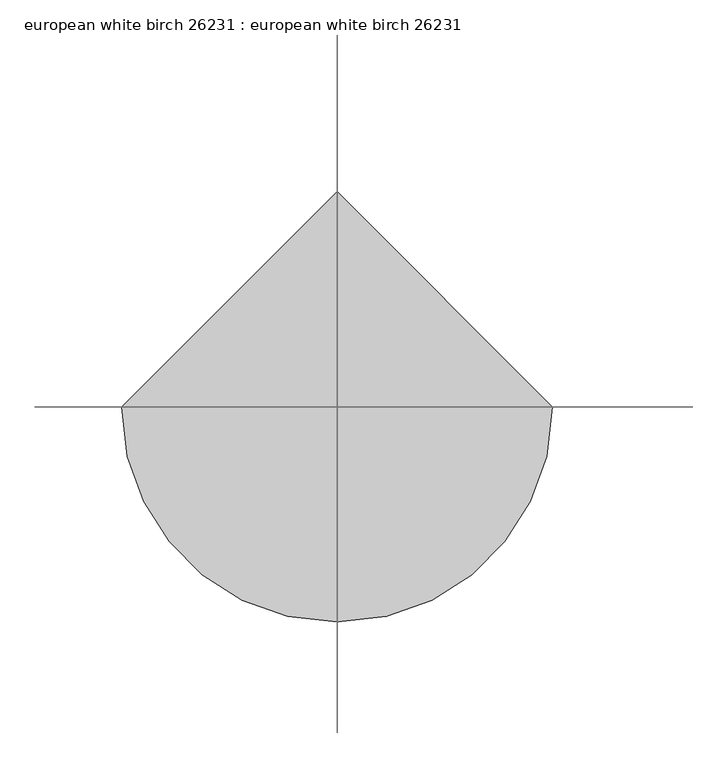
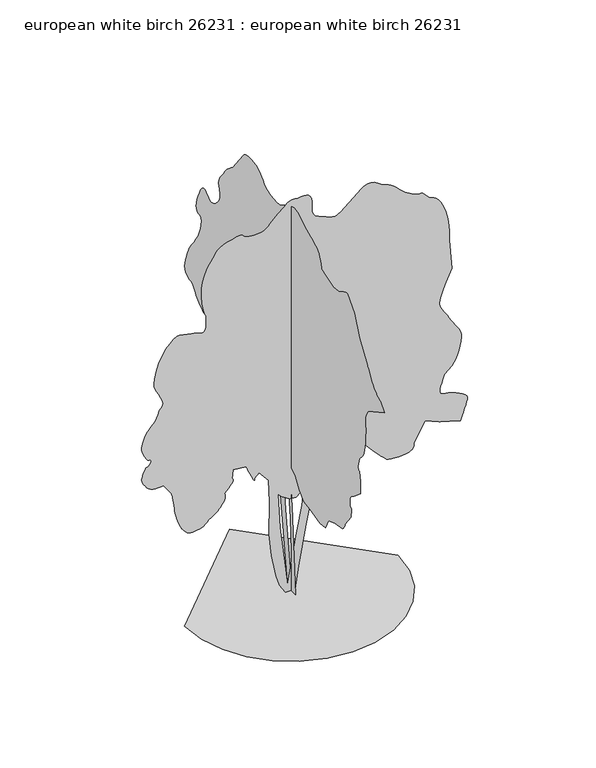
"""IFC4 building model written with IfcOpenShell, lengths in millimetres: proxy geometry, european white birch 26231 : european white birch 26231."""

from ifc_helpers import new_model, si_unit, origin, place, context, project, spatial, triangles, source, transform, mapped, element, save


def european_white_birch_26231_european_white_birch_26231_e71fde4f(model_context):
    return source(origin(), model_context, "Body", "Tessellation", [
        triangles([(27.394651, 0.0040504, 0.0028461), (-40.6021365, 0.0040504, 0.0028461), (-85.9329906, 0.0040461, 71.7768143), (-112.3759078, 0.0040411, 154.8832968), (-146.3742959, 0.004031, 324.873484), (-165.2619874, 0.0040206, 498.6424559), (-161.4844927, 0.004006, 744.1841543), (-169.039464, 0.0039956, 917.9531261), (-237.036004, 0.0039907, 1001.059318), (-271.0331294, 0.0039925, 970.840959), (-270.3066839, 0.0039929, 963.7695883), (-270.075557, 0.0039933, 957.9860023), (-270.8350129, 0.0039934, 954.7830729), (-273.0829134, 0.0039934, 955.4434977), (-277.3120158, 0.0039931, 961.2575323), (-284.0176021, 0.0039923, 973.5155777), (-293.700078, 0.0039911, 993.5053459), (-303.821971, 0.0039898, 1015.3671656), (-311.7620024, 0.0039888, 1032.8676962), (-317.8859382, 0.003988, 1046.7335649), (-322.5544759, 0.0039873, 1057.6911083), (-326.1333272, 0.0039868, 1066.4693516), (-328.985733, 0.0039864, 1073.7921604), (-331.4749343, 0.0039859, 1080.3885601), (-429.6916137, 0.0039853, 1091.7220253), (-437.2481292, 0.0039893, 1023.7262484), (-433.293356, 0.0039894, 1022.0295496), (-429.9024656, 0.0039896, 1019.8705244), (-427.631674, 0.0039898, 1016.7869917), (-427.0500235, 0.00399, 1012.316625), (-428.7111866, 0.0039904, 1005.9945545), (-433.1841331, 0.0039909, 997.3610699), (-441.0251152, 0.0039916, 985.9513739), (-450.1868743, 0.0039923, 973.9905487), (-458.3606123, 0.0039929, 963.8127542), (-465.7062758, 0.0039934, 955.1234591), (-472.3915509, 0.0039939, 947.6228268), (-478.5815437, 0.0039942, 941.0162533), (-484.4387807, 0.0039946, 935.0015768), (-490.1334549, 0.003995, 929.2865913), (-488.5815147, 0.0039955, 919.5735941), (-487.4232642, 0.0039961, 909.8581261), (-487.0600596, 0.0039967, 900.1451288), (-487.8880978, 0.0039973, 890.4322042), (-490.2985611, 0.0039979, 880.7167362), (-494.6927333, 0.0039984, 871.003739), (-501.4669201, 0.003999, 861.2908144), (-508.8125836, 0.0039996, 851.763271), (-515.365781, 0.0040001, 842.4363693), (-522.1831338, 0.0040007, 833.0409399), (-530.3212998, 0.0040013, 823.3152981), (-540.8394442, 0.0040019, 812.9977592), (-554.7941883, 0.0040026, 801.8192265), (-573.2396831, 0.0040033, 789.5154716), (-592.1829672, 0.0040041, 776.4217941), (-607.7557085, 0.0040048, 763.3916302), (-621.2152067, 0.0040056, 750.9583048), (-633.8135656, 0.0040063, 739.6477306), (-646.8107374, 0.0040068, 729.9880732), (-661.4563551, 0.0040073, 722.5103319), (-679.0128416, 0.0040076, 717.742745), (-697.3389759, 0.0040078, 714.6033291), (-713.6812923, 0.0040079, 712.0582083), (-728.3751629, 0.004008, 710.7044392), (-741.7431696, 0.004008, 711.1337008), (-754.1231552, 0.0040078, 713.9429043), (-765.842716, 0.0040075, 719.7239468), (-777.229521, 0.0040069, 729.0736668), (-788.1109062, 0.0040062, 740.6941784), (-798.1336956, 0.0040055, 753.1071562), (-807.361548, 0.0040047, 766.6428125), (-815.8629187, 0.0040037, 781.6313599), (-823.7064079, 0.0040028, 798.4029379), (-830.9530586, 0.0040016, 817.2929186), (-837.6713259, 0.0040004, 838.6238113), (-843.4955343, 0.0039992, 858.8117506), (-848.1996077, 0.0039982, 875.2328413), (-852.042687, 0.0039973, 889.6727303), (-855.291326, 0.0039965, 903.9119774), (-858.2097525, 0.0039955, 919.7387003), (-861.0621946, 0.0039944, 938.9334589), (-864.1127352, 0.0039929, 963.2844435), (-867.2419773, 0.0039915, 988.1637388), (-870.1706503, 0.0039902, 1008.2856211), (-872.9341444, 0.0039893, 1024.4425564), (-875.5681406, 0.0039885, 1037.4270109), (-878.1005442, 0.0039879, 1048.0315235), (-880.566818, 0.0039873, 1057.0510311), (-883.0001724, 0.0039869, 1065.2781452), (-939.6650276, 0.0039821, 1144.6073874), (-960.6453604, 0.0039822, 1143.9037966), (-981.2295691, 0.0039822, 1143.8250223), (-1001.0212389, 0.0039821, 1145.0035841), (-1019.6216297, 0.0039819, 1148.0668419), (-1036.6370882, 0.0039816, 1153.6396122), (-1051.6713449, 0.0039811, 1162.3517984), (-1064.3255871, 0.0039803, 1174.8282898), (-1074.7447186, 0.0039795, 1188.5290524), (-1083.3781305, 0.0039788, 1200.7108669), (-1090.2945688, 0.0039781, 1211.7014025), (-1095.5600178, 0.0039775, 1221.8335602), (-1099.2379183, 0.003977, 1231.4371891), (-1101.3968708, 0.0039764, 1240.842865), (-1102.1004616, 0.0039758, 1250.3805096), (-1100.4266539, 0.0039751, 1261.9120731), (-1096.1086035, 0.0039743, 1276.0193516), (-1090.2056934, 0.0039734, 1291.1195927), (-1083.7743999, 0.0039725, 1305.6229225), (-1077.8714172, 0.0039718, 1317.9470249), (-1073.5534395, 0.0039713, 1326.5043514), (-1071.8795591, 0.0039711, 1329.7098244), (-1068.9941248, 0.003971, 1330.8324303), (-1061.7475468, 0.0039708, 1334.0708954), (-1052.2555389, 0.0039705, 1339.2246506), (-1042.6289463, 0.0039701, 1346.0979229), (-1034.9860989, 0.0039696, 1354.4899979), (-1031.4402397, 0.003969, 1364.2029224), (-1034.1046846, 0.0039684, 1375.0412144), (-1039.5885796, 0.003968, 1382.3080673), (-1043.7516249, 0.0039679, 1383.6975174), (-1047.5844578, 0.0039679, 1382.5722954), (-1052.0777155, 0.003968, 1382.3080673), (-1058.224506, 0.0039677, 1386.2730869), (-1067.012923, 0.003967, 1397.8376427), (-1079.4360746, 0.0039657, 1420.3699883), (-1091.9252106, 0.0039642, 1445.7800652), (-1100.2513739, 0.003963, 1465.4371502), (-1104.4144192, 0.003962, 1481.9243706), (-1104.4144192, 0.0039611, 1497.8171505), (-1100.2513739, 0.00396, 1515.6910595), (-1091.9252106, 0.0039587, 1538.1268993), (-1079.4360746, 0.0039569, 1567.6974781), (-1064.2798777, 0.0039552, 1597.0701038), (-1048.399815, 0.0039538, 1619.0410011), (-1032.4536953, 0.0039528, 1636.3867447), (-1017.0993999, 0.0039519, 1651.8833279), (-1003.0024406, 0.0039509, 1668.3044186), (-990.8230968, 0.0039497, 1688.4261555), (-981.2193953, 0.0039481, 1715.0224972), (-972.0448826, 0.0039467, 1739.5715801), (-961.9458624, 0.0039458, 1754.6033661), (-952.7714224, 0.0039452, 1764.484013), (-946.3731211, 0.0039446, 1773.5695049), (-944.597648, 0.0039439, 1786.2238197), (-949.3017941, 0.0039427, 1806.8080284), (-962.3294146, 0.0039407, 1839.683202), (-979.0807177, 0.0039386, 1873.8004509), (-993.1903942, 0.0039372, 1898.4714741), (-1003.8609638, 0.003936, 1918.5805664), (-1010.3049019, 0.0039348, 1939.0224873), (-1011.7248007, 0.0039332, 1964.6841476), (-1007.3305922, 0.0039311, 2000.4549294), (-996.3298101, 0.0039281, 2051.2269756), (-977.7827591, 0.0039247, 2108.3871494), (-952.959347, 0.0039217, 2159.268346), (-924.3666155, 0.0039191, 2202.6819752), (-894.5216349, 0.003917, 2237.4394466), (-865.9313742, 0.0039155, 2262.3517342), (-841.1054186, 0.0039147, 2276.2302475), (-822.560911, 0.0039146, 2277.8813095), (-705.4567944, 0.0039161, 2251.4372841), (-691.5452162, 0.0039165, 2245.6562416), (-676.5135029, 0.0039168, 2239.8751991), (-661.5453032, 0.003917, 2236.8678246), (-647.8343668, 0.0039169, 2239.4104019), (-636.5669586, 0.0039162, 2250.281686), (-628.9342123, 0.0039149, 2272.2525833), (-626.1275522, 0.0039128, 2308.1021393), (-626.6101536, 0.0039108, 2340.8655464), (-628.1519199, 0.0039099, 2356.9793884), (-630.8849653, 0.0039094, 2364.3021973), (-634.9362442, 0.003909, 2370.7004986), (-640.4429575, 0.0039082, 2384.0379112), (-647.5371466, 0.0039066, 2412.1786354), (-656.3459112, 0.0039035, 2462.9810577), (-661.9085077, 0.0038998, 2524.9316368), (-660.1355782, 0.0038965, 2581.121521), (-652.4800135, 0.0038935, 2631.3882202), (-640.3997915, 0.0038909, 2675.5079109), (-625.3451872, 0.0038886, 2713.2524094), (-608.7691641, 0.0038868, 2744.4943977), (-592.1271203, 0.0038853, 2768.9545326), (-577.5017776, 0.0038841, 2789.7061729), (-564.8602163, 0.0038829, 2809.5183357), (-552.480267, 0.0038818, 2827.9332001), (-538.6474268, 0.0038808, 2844.519397), (-521.6421421, 0.00388, 2858.7688179), (-499.7473303, 0.0038793, 2870.2750923), (-471.2460176, 0.0038788, 2878.5045319), (-442.3357547, 0.0038784, 2885.0579109), (-419.4402045, 0.003878, 2891.1537598), (-401.1674463, 0.0038777, 2895.8528915), (-386.135733, 0.0038776, 2898.2405365), (-372.9506003, 0.0038776, 2897.4022156), (-360.2302649, 0.0038779, 2892.3984512), (-346.5853855, 0.0038786, 2882.2891846), (-328.0611892, 0.0038792, 2871.5959419), (-303.3901842, 0.0038796, 2865.1951698), (-275.2190476, 0.0038797, 2862.7566559), (-246.1878799, 0.0038796, 2863.9757675), (-218.9407967, 0.0038794, 2868.471714), (-196.1211867, 0.0038789, 2875.9392815), (-180.3721843, 0.0038783, 2886.0738373), (-168.3897398, 0.0038776, 2898.2405365), (-155.2838538, 0.0038768, 2911.7277946), (-141.3189358, 0.0038759, 2926.0280846), (-126.7594139, 0.0038751, 2940.5568489), (-111.8694252, 0.0038742, 2954.8571388), (-96.9134068, 0.0038734, 2968.344397), (-82.1555049, 0.0038727, 2980.5110962), (-68.1573178, 0.003872, 2992.5760574), (-54.8202912, 0.0038712, 3005.3776016), (-41.4169714, 0.0038705, 3017.7727753), (-27.2206609, 0.0038698, 3028.6694939), (-11.5045701, 0.0038693, 3036.8989334), (6.4582013, 0.0038691, 3041.3693001), (27.394651, 0.0038691, 3040.9629295), (49.9498399, 0.0038692, 3039.6420799), (71.8443792, 0.0038691, 3040.7344551), (92.4173513, 0.003869, 3041.9535667), (111.007859, 0.0038691, 3041.0390877), (126.954987, 0.0038694, 3035.7812691), (139.5983468, 0.0038701, 3023.8942039), (148.2767597, 0.0038713, 3003.1678528), (152.1975051, 0.0038729, 2976.7517326), (152.8144732, 0.0038745, 2949.9039528), (152.8363106, 0.0038761, 2923.6913086), (154.9729534, 0.0038776, 2899.0276978), (161.9335751, 0.0038789, 2876.9552078), (176.4270581, 0.00388, 2858.4641853), (201.1628484, 0.0038808, 2844.519397), (230.392387, 0.0038815, 2832.759359), (256.9132791, 0.0038822, 2821.2022156), (281.2515464, 0.0038828, 2811.4231613), (303.9388244, 0.0038832, 2804.9971001), (325.5034238, 0.0038833, 2803.5492233), (346.4736554, 0.0038829, 2808.6291458), (367.3752866, 0.0038822, 2821.8626404), (518.4798351, 0.0038745, 2950.2850342), (522.0028032, 0.0038744, 2952.6726791), (531.8706965, 0.003874, 2958.2098412), (547.0243501, 0.0038737, 2964.5597443), (566.409613, 0.0038734, 2969.309745), (588.9648133, 0.0038733, 2970.1224861), (613.6332567, 0.0038737, 2964.5597443), (639.3609015, 0.0038745, 2950.2850342), (662.9625858, 0.0038755, 2934.3845512), (682.9295357, 0.0038761, 2923.8183357), (700.7171127, 0.0038765, 2916.096714), (717.7757372, 0.003877, 2908.7053047), (735.5633869, 0.0038775, 2899.1294357), (755.5303368, 0.0038784, 2884.8800148), (779.1320211, 0.0038797, 2863.4170807), (802.6904669, 0.003881, 2840.7347443), (822.3475519, 0.0038821, 2823.6151497), (839.2969534, 0.0038828, 2810.6612892), (854.7274069, 0.0038834, 2800.5011536), (869.8277206, 0.0038839, 2791.7130272), (885.7865576, 0.0038845, 2782.9246101), (903.7925806, 0.0038851, 2772.7391853), (921.1153605, 0.0038856, 2764.6873512), (935.0701773, 0.0038857, 2761.4360962), (946.9090622, 0.0038858, 2760.445459), (957.8894966, 0.0038859, 2759.1246094), (969.2661278, 0.0038861, 2754.908297), (982.2963644, 0.0038867, 2745.1801117), (998.2323103, 0.0038878, 2727.4000923), (1015.8421366, 0.0038888, 2709.5947838), (1033.1877348, 0.0038895, 2698.6471962), (1050.4673487, 0.00389, 2690.3415985), (1067.8790766, 0.0038906, 2680.4608063), (1085.6209442, 0.0038915, 2664.7382195), (1103.8937387, 0.0038931, 2639.0081039), (1122.890399, 0.0038954, 2598.9776985), (1139.5654713, 0.0038982, 2552.2671776), (1151.2850321, 0.0039008, 2508.9526703), (1158.8719963, 0.0039032, 2468.4345039), (1163.1569818, 0.0039055, 2430.1618401), (1164.9629036, 0.0039077, 2393.5757011), (1165.1152925, 0.0039098, 2358.1121681), (1164.4447666, 0.0039119, 2323.2125542), (1183.3322039, 0.0039254, 2096.5583656), (1160.8760891, 0.0039282, 2049.0019661), (1139.6746943, 0.003931, 2002.6697651), (1120.9853554, 0.0039336, 1958.7811649), (1106.0628651, 0.003936, 1918.5603642), (1096.1619432, 0.0039381, 1883.2289452), (1092.5373825, 0.0039398, 1854.0112518), (1096.4489897, 0.0039411, 1832.1266865), (1105.2043419, 0.0039422, 1814.483868), (1115.1484297, 0.0039432, 1796.9070339), (1126.0856981, 0.0039443, 1778.9975166), (1137.8154327, 0.0039454, 1760.364061), (1150.1394625, 0.0039466, 1740.6053833), (1162.8597616, 0.0039479, 1719.327903), (1175.7782318, 0.0039492, 1696.1351326), (1190.083536, 0.0039507, 1672.4673912), (1206.0423002, 0.003952, 1649.7243027), (1222.0671215, 0.0039534, 1627.4433952), (1236.5705967, 0.0039547, 1605.1651039), (1247.9700462, 0.003956, 1582.42187), (1254.6782124, 0.0039574, 1558.7541286), (1255.1075466, 0.0039589, 1533.6996986), (1250.5482319, 0.0039606, 1505.3836945), (1243.6089752, 0.0039625, 1473.6972565), (1234.6884441, 0.0039645, 1440.8220829), (1224.1805099, 0.0039664, 1408.9400173), (1212.4837675, 0.0039681, 1380.2278164), (1199.9971024, 0.0039695, 1356.867469), (1187.1091536, 0.0039704, 1341.0432896), (1175.1508718, 0.003971, 1330.4793995), (1164.9730774, 0.0039716, 1321.3074303), (1156.2837095, 0.0039721, 1313.2887337), (1148.7831499, 0.0039725, 1306.1970154), (1142.1765764, 0.0039729, 1299.7962433), (1136.1618999, 0.0039732, 1293.8602684), (1130.4468418, 0.0039736, 1288.1553841), (1119.2784828, 0.0039753, 1259.9842838), (1109.1032318, 0.0039769, 1232.7706833), (1100.9092552, 0.0039784, 1207.4723728), (1095.6869722, 0.0039797, 1185.0492502), (1094.4322523, 0.0039808, 1166.4589605), (1098.1329712, 0.0039817, 1152.6591488), (1107.7799114, 0.0039821, 1144.6073874), (1119.8855679, 0.0039824, 1140.5992744), (1130.6017742, 0.0039825, 1137.9779955), (1140.3909296, 0.0039826, 1136.2812241), (1149.7203747, 0.0039827, 1135.0493225), (1159.0472763, 0.0039828, 1133.8148775), (1168.8389751, 0.0039829, 1132.1181787), (1179.5551815, 0.003983, 1129.4968998), (1194.774892, 0.0039834, 1124.1121267), (1215.7451237, 0.0039839, 1115.0925465), (1239.4230389, 0.0039846, 1103.4288689), (1262.7705963, 0.0039854, 1090.1142019), (1282.7503361, 0.0039862, 1076.1391829), (1296.3189846, 0.003987, 1062.4917601), (1300.4363205, 0.0039877, 1050.1676577), (1297.6066967, 0.0039886, 1036.4135553), (1292.5953747, 0.0039897, 1018.2957659), (1285.7677391, 0.0039909, 996.5457127), (1277.4848145, 0.0039924, 971.8848633), (1268.1122761, 0.003994, 945.0472572), (1258.0131832, 0.0039957, 916.7542168), (1247.5510311, 0.0039974, 887.732151), (1088.8924742, 0.0039947, 933.063541), (986.8988451, 0.003992, 978.394931), (903.7925806, 0.0040008, 831.069912), (903.6808142, 0.0040014, 821.3899796), (902.9112391, 0.0040019, 811.9056021), (900.8182709, 0.0040025, 802.8200375), (896.744101, 0.004003, 794.328768), (890.0258337, 0.0040035, 786.6300373), (880.0029716, 0.0040039, 779.9244873), (866.0151627, 0.0040042, 774.4050568), (846.3124409, 0.0040044, 770.254656), (821.2578655, 0.0040046, 767.5546755), (793.3610945, 0.0040047, 766.3761137), (765.1340384, 0.0040046, 766.7850277), (739.086355, 0.0040045, 768.8450037), (717.7325712, 0.0040043, 772.6219534), (703.5797287, 0.004004, 778.1845499), (692.3249651, 0.0040034, 786.972967), (678.2940628, 0.0040027, 799.9244293), (661.9491302, 0.0040017, 816.34552), (643.75511, 0.0040005, 835.5402786), (624.1742558, 0.0039993, 856.8178316), (603.6663142, 0.0039979, 879.4848347), (582.698626, 0.0039965, 902.8426386), (568.1063481, 0.0039956, 918.9335169), (553.3794127, 0.0039947, 934.4301001), (538.3909018, 0.0039938, 948.7353315), (523.0061213, 0.0039931, 961.2575323), (507.0904867, 0.0039924, 971.4022619), (490.5169707, 0.003992, 978.5701384), (473.1484815, 0.0039918, 982.1718807), (299.3795278, 0.0039905, 1004.8388111), (220.0505219, 0.0039938, 948.1740286), (186.0526334, 0.0039972, 891.5117168), (159.6097343, 0.0040064, 736.6301823), (110.5011312, 0.0040218, 479.7550186), (53.8375659, 0.00404, 173.7712428), (-25.4914287, 0.0039615, 56.6666174), (38.7268558, 0.003939, 434.4236286), (80.280474, 0.0039269, 638.4135029), (91.61294, 0.0039203, 747.9636475), (91.61294, 0.0039172, 800.8490095), (68.9477628, 0.0039206, 744.1841543), (34.9493702, 0.0039224, 713.9657953), (-14.1591478, 0.0039219, 721.5197674), (-67.0453035, 0.0039199, 755.5176195), (-97.2657018, 0.0039181, 785.738522), (-82.1555049, 0.0039341, 517.5298568), (0.0001483, 43.8182829, 0.0020761), (0.0001483, -54.3986509, 0.0020703), (0.0001483, -9.0678473, 664.8549122), (0.0001483, 13.5975031, 895.2886665), (0.0001483, 28.7078316, 978.394931), (0.0001483, -54.3986509, 925.5070255), (0.0001483, -107.2847305, 846.1777834), (0.0001483, -163.9485502, 793.292494), (0.0001483, -239.5000614, 778.1820065), (0.0001483, -303.7178349, 763.0715916), (0.0001483, -367.9366259, 747.961104), (0.0001483, -439.7119323, 755.5176195), (0.0001483, -473.7098207, 831.069912), (0.0001483, -556.8160489, 861.288271), (0.0001483, -655.032692, 880.1782516), (0.0001483, -659.8892269, 885.0778799), (0.0001483, -664.7482327, 890.2442797), (0.0001483, -669.6046949, 895.9363741), (0.0001483, -674.4611572, 902.4235508), (0.0001483, -679.3176195, 909.9673491), (0.0001483, -684.1741545, 918.8344677), (0.0001483, -689.0306168, 929.2865913), (0.0001483, -695.1011765, 941.3896317), (0.0001483, -703.3485655, 954.8795786), (0.0001483, -713.4145935, 969.5277397), (0.0001483, -724.9360559, 985.100481), (0.0001483, -737.5445887, 1001.3691828), (0.0001483, -750.8821466, 1018.0976675), (0.0001483, -764.5829092, 1035.0571701), (0.0001483, -772.139352, 1099.2759974), (0.0001483, -766.5208723, 1102.6135843), (0.0001483, -761.2021563, 1106.5454664), (0.0001483, -756.4777353, 1111.6660841), (0.0001483, -752.6449024, 1118.5723486), (0.0001483, -750.0007324, 1127.8560843), (0.0001483, -748.8450617, 1140.1141296), (0.0001483, -749.4724216, 1155.9408525), (0.0001483, -752.3045162, 1171.9860214), (0.0001483, -757.3133675, 1184.861253), (0.0001483, -764.1434738, 1195.0923872), (0.0001483, -772.423855, 1203.2102057), (0.0001483, -781.7964661, 1209.7405483), (0.0001483, -791.8954863, 1215.2142694), (0.0001483, -802.357711, 1220.1596798), (0.0001483, -881.6869532, 1288.1553841), (0.0001483, -885.466519, 1390.1490131), (0.0001483, -870.3560314, 1458.1473335), (0.0001483, -864.7832611, 1459.9406834), (0.0001483, -859.7718664, 1462.7929802), (0.0001483, -855.8831503, 1467.7612816), (0.0001483, -853.6809591, 1475.8994476), (0.0001483, -853.7241251, 1488.266716), (0.0001483, -856.5765673, 1505.922179), (0.0001483, -862.7995886, 1529.9201328), (0.0001483, -870.719236, 1551.8250458), (0.0001483, -878.5043713, 1565.0076714), (0.0001483, -886.4901484, 1573.2347855), (0.0001483, -895.0042362, 1580.2730186), (0.0001483, -904.3742311, 1589.8869667), (0.0001483, -914.9381212, 1605.845731), (0.0001483, -927.0183432, 1631.9137619), (0.0001483, -937.5923344, 1663.1050266), (0.0001483, -944.0667938, 1691.78409), (0.0001483, -947.437373, 1717.7529991), (0.0001483, -948.6921656, 1740.8136555), (0.0001483, -948.8242069, 1760.7704315), (0.0001483, -948.8242069, 1777.4227581), (0.0001483, -949.6852736, 1790.5722462), (0.0001483, -951.4683769, 1799.6908756), (0.0001483, -953.3200081, 1805.7056248), (0.0001483, -954.8389561, 1810.5951519), (0.0001483, -955.6314222, 1816.3430569), (0.0001483, -955.3012098, 1824.9333755), (0.0001483, -953.4521221, 1838.3497078), (0.0001483, -949.6852736, 1858.5705666), (0.0001483, -946.70079, 1881.7531631), (0.0001483, -947.0843422, 1902.9520145), (0.0001483, -950.2796413, 1922.50242), (0.0001483, -955.7203703, 1940.7293598), (0.0001483, -962.8450081, 1957.9658077), (0.0001483, -971.0949406, 1974.53936), (0.0001483, -979.9036325, 1990.7851707), (0.0001483, -1191.4500223, 2107.8892147), (0.0001483, -1138.5621895, 2164.5515991), (0.0001483, -1128.8162001, 2168.6714058), (0.0001483, -1118.8721123, 2173.2205467), (0.0001483, -1108.5292116, 2178.6282108), (0.0001483, -1097.5944866, 2185.3237324), (0.0001483, -1085.8648247, 2193.7387711), (0.0001483, -1073.1445255, 2204.300045), (0.0001483, -1059.2329473, 2217.4395046), (0.0001483, -1043.7160892, 2235.2574577), (0.0001483, -1027.1399935, 2257.7696011), (0.0001483, -1010.7646849, 2282.2627281), (0.0001483, -995.8421946, 2306.029446), (0.0001483, -983.6273151, 2326.3596004), (0.0001483, -975.3773827, 2340.5455078), (0.0001483, -972.3497332, 2345.8770138), (0.0001483, -870.3560314, 2496.9789825), (0.0001483, -809.9142265, 2651.8605171), (0.0001483, -715.4745695, 2746.297776), (0.0001483, -714.1080105, 2746.4248032), (0.0001483, -710.0998976, 2746.4248032), (0.0001483, -703.5797287, 2745.7135094), (0.0001483, -694.6820887, 2743.6560768), (0.0001483, -683.5366207, 2739.6938187), (0.0001483, -670.2752209, 2733.2165977), (0.0001483, -655.032692, 2723.6410194), (0.0001483, -638.8427645, 2713.734938), (0.0001483, -622.6553804, 2706.4196869), (0.0001483, -606.4653803, 2701.2380264), (0.0001483, -590.2754528, 2697.7835861), (0.0001483, -574.085489, 2695.5994171), (0.0001483, -557.8955252, 2694.3038567), (0.0001483, -541.7055977, 2693.4149574), (0.0001483, -447.265868, 2716.071714), (0.0001483, -390.6035926, 2734.9693977), (0.0001483, -389.2700984, 2739.8714241), (0.0001483, -385.4931124, 2752.9017334), (0.0001483, -379.6003035, 2771.5453629), (0.0001483, -371.9244275, 2793.2876404), (0.0001483, -362.7931171, 2815.6397644), (0.0001483, -352.541708, 2836.0611923), (0.0001483, -341.4952529, 2852.0631226), (0.0001483, -328.1907234, 2864.4077179), (0.0001483, -311.3835734, 2875.7360962), (0.0001483, -291.7366622, 2886.4549187), (0.0001483, -269.9079074, 2896.995845), (0.0001483, -246.5594779, 2907.7399567), (0.0001483, -222.3522709, 2919.068335), (0.0001483, -197.946693, 2931.4129303), (0.0001483, -172.8141609, 2945.8655365), (0.0001483, -146.2940319, 2961.968914), (0.0001483, -118.8488412, 2977.6915009), (0.0001483, -90.941106, 2990.9502846), (0.0001483, -63.0331211, 2999.7387016), (0.0001483, -35.5879259, 3001.9740303), (0.0001483, -9.0678473, 2995.6241272), (0.0001483, 15.5359294, 2984.4989342), (0.0001483, 37.8929746, 2973.7039536), (0.0001483, 58.5319923, 2963.1121582), (0.0001483, 77.9815228, 2952.5709412), (0.0001483, 96.7704014, 2941.9791458), (0.0001483, 115.4269479, 2931.1841652), (0.0001483, 134.479991, 2920.0589722), (0.0001483, 158.8525495, 2912.4135086), (0.0001483, 190.6921939, 2911.194397), (0.0001483, 226.364199, 2914.9028915), (0.0001483, 262.2345749, 2922.1416939), (0.0001483, 294.6678241, 2931.4129303), (0.0001483, 320.0322461, 2941.2681427), (0.0001483, 334.690581, 2950.2850342), (0.0001483, 345.0334454, 2961.4610962), (0.0001483, 359.6029049, 2977.2598412), (0.0001483, 378.0077408, 2995.3953621), (0.0001483, 399.8466331, 3013.5055939), (0.0001483, 424.7259284, 3029.3043388), (0.0001483, 452.246814, 3040.4804008), (0.0001483, 482.0181436, 3044.7222931), (0.0001483, 509.7701923, 3045.6111923), (0.0001483, 532.4371227, 3047.2366745), (0.0001483, 551.4007545, 3047.9988373), (0.0001483, 568.0530084, 3046.3224861), (0.0001483, 583.7806821, 3040.607428), (0.0001483, 599.9706096, 3029.2534698), (0.0001483, 618.0096611, 3010.7368675), (0.0001483, 742.6702932, 2848.3040497), (0.0001483, 753.8818909, 2837.2805946), (0.0001483, 767.6029284, 2826.4091652), (0.0001483, 783.1096127, 2814.9031815), (0.0001483, 799.6755346, 2801.8981613), (0.0001483, 816.5690529, 2786.683683), (0.0001483, 833.0663017, 2768.3955551), (0.0001483, 848.4409447, 2746.297776), (0.0001483, 862.736075, 2724.5807877), (0.0001483, 876.3047235, 2707.0801117), (0.0001483, 888.8828075, 2692.4751892), (0.0001483, 900.2035555, 2679.4704597), (0.0001483, 910.0054281, 2666.7194939), (0.0001483, 918.0241974, 2652.9273125), (0.0001483, 923.9932371, 2636.7474861), (0.0001483, 925.4028894, 2616.8085869), (0.0001483, 921.857103, 2593.3896675), (0.0001483, 916.2614416, 2567.5581047), (0.0001483, 911.5269196, 2540.4815598), (0.0001483, 910.5566299, 2513.2907776), (0.0001483, 916.2614416, 2487.0781334), (0.0001483, 931.5471365, 2462.9810577), (0.0001483, 951.2956404, 2442.8058357), (0.0001483, 968.7962437, 2427.385556), (0.0001483, 984.5772572, 2416.3949478), (0.0001483, 999.1695351, 2409.5014732), (0.0001483, 1013.1014608, 2406.3721584), (0.0001483, 1026.9012726, 2406.6820232), (0.0001483, 1041.0973537, 2410.0957684), (0.0001483, 1055.7023489, 2418.4549965), (0.0001483, 1070.502899, 2431.1752956), (0.0001483, 1085.7022619, 2444.2917915), (0.0001483, 1101.4959927, 2453.8397552), (0.0001483, 1118.0821169, 2455.8564926), (0.0001483, 1135.658951, 2446.3745132), (0.0001483, 1154.424448, 2421.4292336), (0.0001483, 1172.6082945, 2386.9666569), (0.0001483, 1187.9498726, 2352.5064056), (0.0001483, 1199.9209442, 2319.4331337), (0.0001483, 1207.9930532, 2289.1360004), (0.0001483, 1211.640505, 2263.0019852), (0.0001483, 1210.3298292, 2242.4177765), (0.0001483, 1203.5327877, 2228.7729698), (0.0001483, 1192.4761951, 2222.4051899), (0.0001483, 1179.8345976, 2220.4010971), (0.0001483, 1167.2565136, 2219.2555275), (0.0001483, 1156.3980194, 2215.468404), (0.0001483, 1148.9075609, 2205.5344173), (0.0001483, 1146.4412144, 2185.9510197), (0.0001483, 1150.6474983, 2153.2206047), (0.0001483, 1159.9972183, 2115.6438286), (0.0001483, 1171.3306835, 2083.4164352), (0.0001483, 1183.8528843, 2055.8852669), (0.0001483, 1196.7713545, 2032.382777), (0.0001483, 1209.2934826, 2012.2481049), (0.0001483, 1220.6269478, 1994.8263485), (0.0001483, 1229.9766678, 1979.4517056), (0.0001483, 1240.3526333, 1963.1729027), (0.0001483, 1254.2286758, 1944.0543022), (0.0001483, 1270.0223339, 1922.9544273), (0.0001483, 1286.1462044, 1900.7294758), (0.0001483, 1301.0128841, 1878.2402962), (0.0001483, 1313.0397663, 1856.345557), (0.0001483, 1320.6394478, 1835.9036362), (0.0001483, 1327.6548626, 1813.7878349), (0.0001483, 1337.4440907, 1787.5776615), (0.0001483, 1347.6981159, 1759.1854992), (0.0001483, 1356.1029808, 1730.5292542), (0.0001483, 1360.3421116, 1703.5239258), (0.0001483, 1358.1069283, 1680.0874203), (0.0001483, 1347.0808571, 1662.134737), (0.0001483, 1331.1449112, 1650.1204994), (0.0001483, 1315.8032604, 1642.3328934), (0.0001483, 1301.1881641, 1637.45354), (0.0001483, 1287.4340618, 1634.1617352), (0.0001483, 1274.6679806, 1631.134013), (0.0001483, 1263.0272667, 1627.0471985), (0.0001483, 1252.6411274, 1620.5829128), (0.0001483, 1244.3708473, 1612.653019), (0.0001483, 1238.27994, 1604.7891094), (0.0001483, 1233.3142548, 1596.5951328), (0.0001483, 1228.4120831, 1587.6746017), (0.0001483, 1222.5218903, 1577.628994), (0.0001483, 1214.5792791, 1566.066909), (0.0001483, 1203.5327877, 1552.5845924), (0.0001483, 1190.6930918, 1539.1175365), (0.0001483, 1178.0490234, 1527.6289936), (0.0001483, 1165.5699886, 1517.7941288), (0.0001483, 1153.2256113, 1509.2801136), (0.0001483, 1140.9777397, 1501.7592064), (0.0001483, 1128.7983959, 1494.8985786), (0.0001483, 1116.6495735, 1488.3656925), (0.0001483, 1094.9198679, 1495.4802292), (0.0001483, 1073.9521797, 1501.5711365), (0.0001483, 1054.5008961, 1505.6149303), (0.0001483, 1037.3305052, 1506.5826038), (0.0001483, 1023.200481, 1503.4559052), (0.0001483, 1012.8702976, 1495.2059727), (0.0001483, 1007.0994289, 1480.8117931), (0.0001483, 1005.2935072, 1464.103656), (0.0001483, 1006.0656258, 1449.3792641), (0.0001483, 1008.9841249, 1436.3059341), (0.0001483, 1013.6195978, 1424.5559246), (0.0001483, 1019.5453989, 1413.7964069), (0.0001483, 1026.3297958, 1403.6974594), (0.0001483, 1033.5433817, 1393.9285789), (0.0001483, 1045.6134298, 1385.8005867), (0.0001483, 1057.2542891, 1377.4744961), (0.0001483, 1068.0365524, 1368.7520634), (0.0001483, 1077.5311037, 1359.4328648), (0.0001483, 1085.3059925, 1349.3235981), (0.0001483, 1090.934646, 1338.2213688), (0.0001483, 1093.9851866, 1325.9302586), (0.0001483, 1099.3597858, 1310.8528358), (0.0001483, 1110.6145494, 1292.2753361), (0.0001483, 1125.3058765, 1271.3152782), (0.0001483, 1140.9878408, 1249.1029713), (0.0001483, 1155.2194576, 1226.7560795), (0.0001483, 1165.549641, 1205.402223), (0.0001483, 1169.5349356, 1186.161755), (0.0001483, 1170.7134974, 1164.7850801), (0.0001483, 1173.4134779, 1137.7239412), (0.0001483, 1176.3751431, 1107.1627253), (0.0001483, 1178.346171, 1075.2781162), (0.0001483, 1178.0718418, 1044.2545738), (0.0001483, 1174.2923487, 1016.2688547), (0.0001483, 1165.7579132, 993.5053459), (0.0001483, 1155.8900562, 976.9065044), (0.0001483, 1148.3360842, 965.2656452), (0.0001483, 1142.1664026, 957.5237486), (0.0001483, 1136.461591, 952.6240477), (0.0001483, 1130.2944529, 949.5049793), (0.0001483, 1122.7404808, 947.1173344), (0.0001483, 1112.8726238, 944.3970062), (0.0001483, 1102.430674, 943.3505585), (0.0001483, 1093.6422569, 945.275877), (0.0001483, 1086.3067308, 948.0622622), (0.0001483, 1080.2285408, 949.5938547), (0.0001483, 1075.2069723, 947.7548681), (0.0001483, 1071.043927, 940.4320593), (0.0001483, 1067.5412338, 925.5070255), (0.0001483, 1064.4805195, 907.1809639), (0.0001483, 1061.5493757, 890.8385748), (0.0001483, 1058.422677, 876.1472477), (0.0001483, 1054.7650515, 862.7766975), (0.0001483, 1050.2489754, 850.3967119), (0.0001483, 1044.544091, 838.6796946), (0.0001483, 1037.3203314, 827.2903461), (0.0001483, 1027.9045544, 814.7808626), (0.0001483, 1016.1088354, 800.7498877), (0.0001483, 1002.331842, 786.45483), (0.0001483, 986.9673729, 773.1502642), (0.0001483, 970.4142408, 762.0911282), (0.0001483, 953.0685699, 754.5371561), (0.0001483, 935.3267023, 751.7406698), (0.0001483, 913.4547815, 757.3895983), (0.0001483, 885.700153, 771.9590578), (0.0001483, 855.4360846, 791.882769), (0.0001483, 826.0305393, 813.5895836), (0.0001483, 800.8540237, 833.5133675), (0.0001483, 783.2747189, 848.0853704), (0.0001483, 776.668218, 853.7342989), (0.0001483, 772.4619341, 859.0429138), (0.0001483, 761.5145645, 872.1493086), (0.0001483, 746.3380926, 888.8218374), (0.0001483, 729.4419582, 904.8365576), (0.0001483, 713.3409061, 915.9592072), (0.0001483, 700.5444489, 917.9632273), (0.0001483, 693.5619535, 906.6195883), (0.0001483, 693.1657568, 889.1647671), (0.0001483, 696.8639322, 874.2854427), (0.0001483, 702.2843136, 859.9344292), (0.0001483, 707.0417267, 844.0645403), (0.0001483, 708.758773, 824.6259012), (0.0001483, 705.0579815, 799.5713259), (0.0001483, 693.5619535, 766.8510847), (0.0001483, 679.8942558, 733.8209787), (0.0001483, 670.2574894, 708.4565386), (0.0001483, 663.1302355, 689.6351583), (0.0001483, 656.9961622, 676.2315434), (0.0001483, 650.3337055, 667.1230877), (0.0001483, 641.6215193, 661.1871128), (0.0001483, 629.343199, 657.3009401), (0.0001483, 615.6627113, 655.8125135), (0.0001483, 603.6383726, 657.4329815), (0.0001483, 593.0643451, 661.5630346), (0.0001483, 583.7476536, 667.6082325), (0.0001483, 575.4875836, 674.9768234), (0.0001483, 568.0860005, 683.0717508), (0.0001483, 561.3448422, 691.2987923), (0.0001483, 555.7517607, 702.0354189), (0.0001483, 551.7436478, 717.5319294), (0.0001483, 549.0563481, 736.9933868), (0.0001483, 547.4256701, 759.6247816), (0.0001483, 546.5874581, 784.636191), (0.0001483, 546.2801368, 811.23246), (0.0001483, 546.2369345, 838.6238113), (0.0001483, 553.7909065, 970.8384155), (0.0001483, 602.8992462, 1099.2759974), (0.0001483, 504.6825668, 1186.161755), (0.0001483, 357.3575478, 1193.715727), (0.0001483, 285.5822413, 1103.052947), (0.0001483, 194.9212963, 1016.1698055), (0.0001483, 164.7003938, 876.3986858), (0.0001483, 138.2574766, 664.8549122), (0.0002414, 85.3713969, 989.7258528), (0.0002414, 58.9284843, 936.8404907), (0.0002414, 32.4853173, 793.292494), (0.0002414, 6.0423779, 559.0842607), (0.0002414, -1.5127294, 309.7630328), (0.0002414, 2.264719, 75.5535415), (0.0002414, 70.2612001, 593.0821492), (0.0002414, 126.9247654, 1035.0571701), (-787.0034157, 0.0, 8.68e-05), (-766.1982903, -180.3292545, 7.6e-05), (-706.9426775, -345.9326274, 6.61e-05), (-613.9838167, -492.0663674, 5.74e-05), (-492.0663674, -613.9838167, 5.02e-05), (-345.9326274, -706.9426775, 4.46e-05), (-180.3290002, -766.1982903, 4.11e-05), (3.45e-05, -787.0034157, 3.99e-05), (180.3292545, -766.1982903, 4.11e-05), (345.9326274, -706.9426775, 4.46e-05), (492.0663674, -613.9838167, 5.02e-05), (613.9838167, -492.0663674, 5.74e-05), (706.9426775, -345.9326274, 6.61e-05), (766.1982903, -180.3290002, 7.6e-05), (787.0034157, 6.88e-05, 8.68e-05), (-0.0001035, 787.0034157, 0.0001337)], [[383, 1, 2], [383, 2, 3], [382, 1, 383], [382, 383, 384], [381, 382, 384], [381, 384, 385], [380, 381, 385], [380, 385, 386], [393, 383, 3], [393, 3, 4], [393, 4, 5], [393, 5, 6], [393, 6, 7], [392, 393, 7], [392, 7, 8], [12, 13, 14], [12, 14, 15], [11, 12, 15], [379, 380, 386], [379, 386, 387], [344, 345, 346], [11, 15, 16], [10, 11, 16], [343, 344, 346], [342, 343, 346], [341, 342, 346], [340, 341, 346], [9, 10, 16], [9, 16, 17], [9, 17, 18], [9, 18, 19], [339, 340, 346], [338, 339, 346], [337, 338, 346], [336, 337, 346], [335, 336, 346], [334, 335, 346], [333, 334, 346], [332, 333, 346], [331, 332, 346], [330, 331, 346], [329, 330, 346], [328, 329, 346], [327, 328, 346], [327, 346, 347], [326, 327, 347], [325, 326, 347], [324, 325, 347], [323, 324, 347], [388, 389, 390], [387, 388, 390], [387, 390, 391], [387, 391, 392], [387, 392, 8], [379, 387, 8], [378, 379, 8], [378, 8, 9], [322, 323, 347], [9, 19, 20], [377, 378, 9], [110, 111, 112], [9, 20, 21], [121, 122, 123], [120, 121, 123], [120, 123, 124], [9, 21, 22], [377, 9, 22], [377, 22, 23], [377, 23, 24], [281, 282, 283], [120, 124, 125], [28, 29, 30], [27, 28, 30], [27, 30, 31], [26, 27, 31], [26, 31, 32], [26, 32, 33], [26, 33, 34], [119, 120, 125], [321, 322, 347], [221, 222, 223], [221, 223, 224], [220, 221, 224], [220, 224, 225], [219, 220, 225], [219, 225, 226], [218, 219, 226], [218, 226, 227], [217, 218, 227], [217, 227, 228], [216, 217, 228], [215, 216, 228], [214, 215, 228], [213, 214, 228], [212, 213, 228], [211, 212, 228], [210, 211, 228], [209, 210, 228], [208, 209, 228], [208, 228, 229], [207, 208, 229], [206, 207, 229], [205, 206, 229], [204, 205, 229], [203, 204, 229], [203, 229, 230], [202, 203, 230], [202, 230, 231], [26, 34, 35], [158, 159, 160], [158, 160, 161], [157, 158, 161], [156, 157, 161], [155, 156, 161], [154, 155, 161], [154, 161, 162], [154, 162, 163], [153, 154, 163], [152, 153, 163], [152, 163, 164], [151, 152, 164], [150, 151, 164], [149, 150, 164], [148, 149, 164], [147, 148, 164], [146, 147, 164], [145, 146, 164], [144, 145, 164], [144, 164, 165], [143, 144, 165], [281, 283, 284], [201, 202, 231], [26, 35, 36], [119, 125, 126], [109, 110, 112], [109, 112, 113], [108, 109, 113], [108, 113, 114], [107, 108, 114], [26, 36, 37], [201, 231, 232], [201, 232, 233], [281, 284, 285], [25, 26, 37], [25, 37, 38], [25, 38, 39], [25, 39, 40], [193, 194, 195], [193, 195, 196], [192, 193, 196], [191, 192, 196], [191, 196, 197], [190, 191, 197], [189, 190, 197], [188, 189, 197], [187, 188, 197], [186, 187, 197], [185, 186, 197], [184, 185, 197], [183, 184, 197], [182, 183, 197], [182, 197, 198], [181, 182, 198], [180, 181, 198], [179, 180, 198], [178, 179, 198], [177, 178, 198], [176, 177, 198], [175, 176, 198], [175, 198, 199], [174, 175, 199], [173, 174, 199], [172, 173, 199], [171, 172, 199], [170, 171, 199], [170, 199, 200], [170, 200, 201], [170, 201, 233], [169, 170, 233], [168, 169, 233], [167, 168, 233], [167, 233, 234], [167, 234, 235], [166, 167, 235], [166, 235, 236], [106, 107, 114], [106, 114, 115], [105, 106, 115], [104, 105, 115], [103, 104, 115], [102, 103, 115], [101, 102, 115], [100, 101, 115], [99, 100, 115], [98, 99, 115], [97, 98, 115], [96, 97, 115], [95, 96, 115], [94, 95, 115], [93, 94, 115], [92, 93, 115], [91, 92, 115], [90, 91, 115], [90, 115, 116], [90, 116, 117], [119, 126, 127], [119, 127, 128], [119, 128, 129], [119, 129, 130], [119, 130, 131], [119, 131, 132], [119, 132, 133], [119, 133, 134], [119, 134, 135], [119, 135, 136], [118, 119, 136], [118, 136, 137], [118, 137, 138], [117, 118, 138], [90, 117, 138], [89, 90, 138], [89, 138, 139], [89, 139, 140], [89, 140, 141], [89, 141, 142], [89, 142, 143], [89, 143, 165], [89, 165, 166], [89, 166, 236], [88, 89, 236], [87, 88, 236], [86, 87, 236], [85, 86, 236], [84, 85, 236], [84, 236, 237], [83, 84, 237], [82, 83, 237], [81, 82, 237], [80, 81, 237], [79, 80, 237], [78, 79, 237], [77, 78, 237], [76, 77, 237], [75, 76, 237], [74, 75, 237], [73, 74, 237], [72, 73, 237], [71, 72, 237], [70, 71, 237], [69, 70, 237], [68, 69, 237], [67, 68, 237], [66, 67, 237], [65, 66, 237], [64, 65, 237], [63, 64, 237], [62, 63, 237], [61, 62, 237], [60, 61, 237], [59, 60, 237], [58, 59, 237], [57, 58, 237], [56, 57, 237], [55, 56, 237], [54, 55, 237], [54, 237, 238], [361, 362, 363], [360, 361, 363], [360, 363, 364], [359, 360, 364], [359, 364, 365], [358, 359, 365], [358, 365, 366], [357, 358, 366], [356, 357, 366], [355, 356, 366], [354, 355, 366], [353, 354, 366], [352, 353, 366], [351, 352, 366], [350, 351, 366], [349, 350, 366], [348, 349, 366], [347, 348, 366], [347, 366, 367], [347, 367, 368], [347, 368, 369], [347, 369, 370], [347, 370, 371], [321, 347, 371], [321, 371, 372], [321, 372, 373], [320, 321, 373], [320, 373, 374], [319, 320, 374], [319, 374, 375], [318, 319, 375], [317, 318, 375], [317, 375, 376], [317, 376, 377], [316, 317, 377], [316, 377, 24], [315, 316, 24], [314, 315, 24], [313, 314, 24], [312, 313, 24], [311, 312, 24], [310, 311, 24], [309, 310, 24], [308, 309, 24], [307, 308, 24], [306, 307, 24], [305, 306, 24], [304, 305, 24], [303, 304, 24], [302, 303, 24], [301, 302, 24], [300, 301, 24], [299, 300, 24], [298, 299, 24], [297, 298, 24], [296, 297, 24], [295, 296, 24], [294, 295, 24], [293, 294, 24], [292, 293, 24], [291, 292, 24], [290, 291, 24], [289, 290, 24], [288, 289, 24], [287, 288, 24], [286, 287, 24], [285, 286, 24], [281, 285, 24], [280, 281, 24], [279, 280, 24], [278, 279, 24], [277, 278, 24], [276, 277, 24], [275, 276, 24], [274, 275, 24], [273, 274, 24], [272, 273, 24], [271, 272, 24], [270, 271, 24], [269, 270, 24], [268, 269, 24], [267, 268, 24], [266, 267, 24], [265, 266, 24], [264, 265, 24], [263, 264, 24], [262, 263, 24], [261, 262, 24], [260, 261, 24], [259, 260, 24], [258, 259, 24], [257, 258, 24], [256, 257, 24], [255, 256, 24], [254, 255, 24], [253, 254, 24], [252, 253, 24], [251, 252, 24], [250, 251, 24], [249, 250, 24], [248, 249, 24], [247, 248, 24], [246, 247, 24], [245, 246, 24], [244, 245, 24], [243, 244, 24], [242, 243, 24], [241, 242, 24], [240, 241, 24], [239, 240, 24], [238, 239, 24], [238, 24, 25], [54, 238, 25], [54, 25, 40], [53, 54, 40], [52, 53, 40], [51, 52, 40], [50, 51, 40], [49, 50, 40], [48, 49, 40], [48, 40, 41], [47, 48, 41], [47, 41, 42], [47, 42, 43], [46, 47, 43], [45, 46, 43], [44, 45, 43], [764, 394, 770], [764, 770, 771], [764, 771, 772], [763, 764, 772], [762, 763, 772], [770, 394, 395], [770, 395, 396], [769, 770, 396], [768, 769, 396], [767, 768, 396], [767, 396, 397], [766, 767, 397], [766, 397, 398], [765, 766, 398], [475, 476, 477], [475, 477, 478], [475, 478, 479], [475, 479, 480], [475, 480, 481], [475, 481, 482], [475, 482, 483], [475, 483, 484], [422, 423, 424], [475, 484, 485], [404, 405, 406], [439, 440, 441], [761, 762, 772], [422, 424, 425], [403, 404, 406], [475, 485, 486], [437, 438, 439], [650, 651, 652], [439, 441, 442], [437, 439, 442], [436, 437, 442], [436, 442, 443], [435, 436, 443], [475, 486, 487], [421, 422, 425], [421, 425, 426], [493, 494, 495], [493, 495, 496], [493, 496, 497], [493, 497, 498], [493, 498, 499], [493, 499, 500], [493, 500, 501], [493, 501, 502], [492, 493, 502], [492, 502, 503], [492, 503, 504], [492, 504, 505], [492, 505, 506], [434, 435, 443], [492, 506, 507], [475, 487, 488], [772, 765, 398], [492, 507, 508], [592, 593, 594], [591, 592, 594], [591, 594, 595], [590, 591, 595], [590, 595, 596], [589, 590, 596], [589, 596, 597], [588, 589, 597], [588, 597, 598], [588, 598, 599], [587, 588, 599], [587, 599, 600], [587, 600, 601], [587, 601, 602], [587, 602, 603], [587, 603, 604], [587, 604, 605], [587, 605, 606], [587, 606, 607], [586, 587, 607], [585, 586, 607], [585, 607, 608], [420, 421, 426], [420, 426, 427], [402, 403, 406], [407, 408, 409], [475, 488, 489], [407, 409, 410], [407, 410, 411], [407, 411, 412], [407, 412, 413], [407, 413, 414], [407, 414, 415], [407, 415, 416], [434, 443, 444], [400, 401, 402], [400, 402, 406], [399, 400, 406], [399, 406, 407], [399, 407, 416], [399, 416, 417], [399, 417, 418], [399, 418, 419], [399, 419, 420], [399, 420, 427], [399, 427, 428], [399, 428, 429], [399, 429, 430], [399, 430, 431], [398, 399, 431], [398, 431, 432], [772, 398, 432], [772, 432, 433], [772, 433, 434], [772, 434, 444], [772, 444, 445], [772, 445, 446], [772, 446, 447], [761, 772, 447], [760, 761, 447], [760, 447, 448], [760, 448, 449], [584, 585, 608], [475, 489, 490], [649, 650, 652], [474, 475, 490], [474, 490, 491], [474, 491, 492], [474, 492, 508], [473, 474, 508], [472, 473, 508], [472, 508, 509], [471, 472, 509], [470, 471, 509], [470, 509, 510], [469, 470, 510], [760, 449, 450], [584, 608, 609], [628, 629, 630], [628, 630, 631], [627, 628, 631], [627, 631, 632], [627, 632, 633], [626, 627, 633], [626, 633, 634], [626, 634, 635], [625, 626, 635], [625, 635, 636], [624, 625, 636], [624, 636, 637], [623, 624, 637], [622, 623, 637], [621, 622, 637], [620, 621, 637], [619, 620, 637], [619, 637, 638], [618, 619, 638], [617, 618, 638], [617, 638, 639], [616, 617, 639], [616, 639, 640], [615, 616, 640], [614, 615, 640], [614, 640, 641], [614, 641, 642], [614, 642, 643], [614, 643, 644], [614, 644, 645], [614, 645, 646], [614, 646, 647], [614, 647, 648], [614, 648, 649], [614, 649, 652], [614, 652, 653], [614, 653, 654], [614, 654, 655], [614, 655, 656], [613, 614, 656], [612, 613, 656], [611, 612, 656], [611, 656, 657], [610, 611, 657], [609, 610, 657], [584, 609, 657], [583, 584, 657], [582, 583, 657], [581, 582, 657], [580, 581, 657], [580, 657, 658], [468, 469, 510], [713, 714, 715], [712, 713, 715], [712, 715, 716], [711, 712, 716], [710, 711, 716], [710, 716, 717], [709, 710, 717], [708, 709, 717], [707, 708, 717], [707, 717, 718], [706, 707, 718], [705, 706, 718], [704, 705, 718], [703, 704, 718], [702, 703, 718], [701, 702, 718], [701, 718, 719], [700, 701, 719], [700, 719, 720], [699, 700, 720], [699, 720, 721], [699, 721, 722], [699, 722, 723], [699, 723, 724], [699, 724, 725], [698, 699, 725], [698, 725, 726], [760, 450, 451], [760, 451, 452], [760, 452, 453], [760, 453, 454], [760, 454, 455], [760, 455, 456], [760, 456, 457], [760, 457, 458], [760, 458, 459], [760, 459, 460], [760, 460, 461], [760, 461, 462], [760, 462, 463], [760, 463, 464], [760, 464, 465], [760, 465, 466], [760, 466, 467], [760, 467, 468], [760, 468, 510], [759, 760, 510], [759, 510, 511], [759, 511, 512], [759, 512, 513], [759, 513, 514], [759, 514, 515], [759, 515, 516], [759, 516, 517], [759, 517, 518], [759, 518, 519], [759, 519, 520], [759, 520, 521], [759, 521, 522], [759, 522, 523], [759, 523, 524], [759, 524, 525], [759, 525, 526], [759, 526, 527], [759, 527, 528], [759, 528, 529], [759, 529, 530], [759, 530, 531], [759, 531, 532], [759, 532, 533], [759, 533, 534], [759, 534, 535], [759, 535, 536], [759, 536, 537], [759, 537, 538], [759, 538, 539], [759, 539, 540], [759, 540, 541], [759, 541, 542], [759, 542, 543], [759, 543, 544], [759, 544, 545], [759, 545, 546], [759, 546, 547], [759, 547, 548], [759, 548, 549], [759, 549, 550], [759, 550, 551], [759, 551, 552], [759, 552, 553], [759, 553, 554], [759, 554, 555], [759, 555, 556], [759, 556, 557], [759, 557, 558], [759, 558, 559], [759, 559, 560], [759, 560, 561], [759, 561, 562], [759, 562, 563], [759, 563, 564], [759, 564, 565], [759, 565, 566], [759, 566, 567], [759, 567, 568], [759, 568, 569], [759, 569, 570], [759, 570, 571], [759, 571, 572], [759, 572, 573], [759, 573, 574], [759, 574, 575], [759, 575, 576], [759, 576, 577], [759, 577, 578], [759, 578, 579], [759, 579, 580], [759, 580, 658], [759, 658, 659], [759, 659, 660], [758, 759, 660], [758, 660, 661], [758, 661, 662], [758, 662, 663], [758, 663, 664], [758, 664, 665], [758, 665, 666], [758, 666, 667], [758, 667, 668], [758, 668, 669], [758, 669, 670], [758, 670, 671], [758, 671, 672], [758, 672, 673], [758, 673, 674], [758, 674, 675], [758, 675, 676], [758, 676, 677], [758, 677, 678], [758, 678, 679], [758, 679, 680], [758, 680, 681], [758, 681, 682], [758, 682, 683], [758, 683, 684], [758, 684, 685], [758, 685, 686], [758, 686, 687], [758, 687, 688], [758, 688, 689], [758, 689, 690], [758, 690, 691], [758, 691, 692], [758, 692, 693], [758, 693, 694], [739, 740, 741], [739, 741, 742], [738, 739, 742], [738, 742, 743], [738, 743, 744], [738, 744, 745], [738, 745, 746], [738, 746, 747], [737, 738, 747], [737, 747, 748], [737, 748, 749], [737, 749, 750], [737, 750, 751], [737, 751, 752], [736, 737, 752], [736, 752, 753], [735, 736, 753], [735, 753, 754], [735, 754, 755], [734, 735, 755], [733, 734, 755], [733, 755, 756], [732, 733, 756], [731, 732, 756], [730, 731, 756], [730, 756, 757], [729, 730, 757], [728, 729, 757], [728, 757, 758], [727, 728, 758], [726, 727, 758], [698, 726, 758], [697, 698, 758], [694, 695, 696], [758, 694, 696], [697, 758, 696], [787, 788, 773], [786, 787, 773], [786, 773, 774], [785, 786, 774], [785, 774, 775], [785, 775, 776], [784, 785, 776], [783, 784, 776], [783, 776, 777], [783, 777, 778], [783, 778, 779], [783, 779, 780], [783, 780, 781], [783, 781, 782]], closed=False),
    ])


if __name__ == "__main__":
    model = new_model("IFC4")
    model_context = context("Model", 3, world=origin())
    ifc_project = project(units=[si_unit("LENGTHUNIT", "METRE", prefix="MILLI")], contexts=[model_context])
    site = spatial("IfcSite", under=ifc_project)
    building = spatial("IfcBuilding", under=site)
    placement = place(None, origin())
    european_white_birch_26231_european_white_birch_26231_shape = european_white_birch_26231_european_white_birch_26231_e71fde4f(model_context)
    element("IfcBuildingElementProxy", 1, Name="european white birch 26231 : european white birch 26231", ObjectType="european white birch 26231 : european white birch 26231", at=placement, inside=building, context=model_context, shape_type="MappedRepresentation", body=[
        mapped(european_white_birch_26231_european_white_birch_26231_shape, transform((0.0, 0.0, 0.0), x_axis=(1.0, 0.0, 0.0), y_axis=(0.0, 1.0, 0.0), z_axis=(0.0, 0.0, 1.0))),
    ])
    save(model, "model.ifc")

# Revit data of these elements
# Type "european white birch 26231 : european white birch 26231"
#   built-in parameter 1005195 = "RPC-8-G3GH-G6G0-PPM0-L"
#   Height = 0
